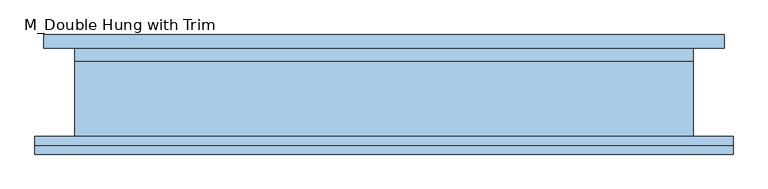
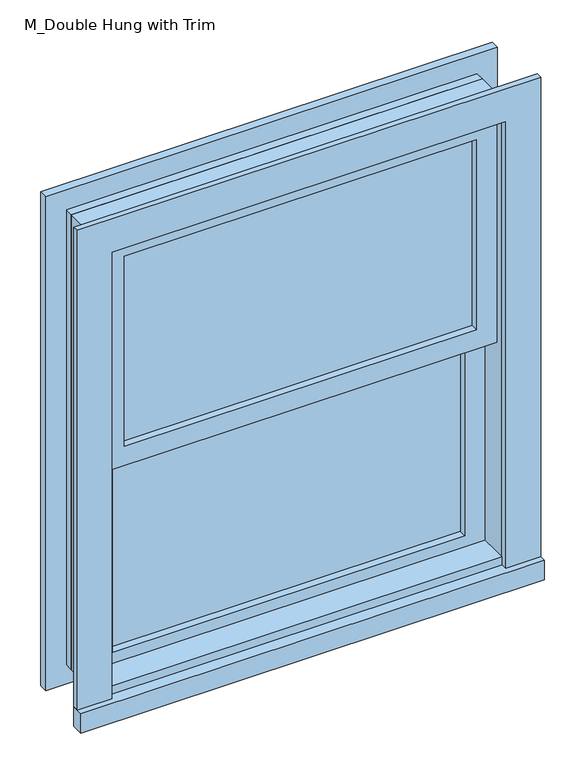
"""IFC4 building model written with IfcOpenShell, lengths in millimetres: window geometry, M_Double Hung with Trim."""

from ifc_helpers import new_model, si_unit, frame, origin, place, context, project, spatial, polyline, outline, extrude, source, transform, mapped, element, save


def m_double_hung_with_trim_e19062af(model_context):
    return source(origin(), model_context, "Body", "SweptSolid", [
        extrude(outline(polyline([(-381.0, 15.825), (-381.0, 28.525), (381.0, 28.525), (381.0, 15.825), (-381.0, 15.825)])), frame((0.0, 0.0, 628.65), z_axis=(0.0, 0.0, 1.0), x_axis=(1.0, 0.0, 0.0)), (0.0, 0.0, 1.0), 454.025),
        extrude(outline(polyline([(1127.125, -425.45), (584.2, -425.45), (584.2, 425.45), (1127.125, 425.45), (1127.125, -425.45)]), holes=[polyline([(1082.675, -381.0), (1082.675, 381.0), (628.65, 381.0), (628.65, -381.0), (1082.675, -381.0)])]), frame((0.0, -0.05, 0.0), z_axis=(0.0, 1.0, 0.0), x_axis=(0.0, 0.0, 1.0)), (0.0, 0.0, 1.0), 44.45),
        extrude(outline(polyline([(-501.65, -89.2), (-501.65, -63.5), (501.65, -63.5), (501.65, -89.2), (-501.65, -89.2)])), frame((0.0, 0.0, 539.75), z_axis=(0.0, 0.0, 1.0), x_axis=(1.0, 0.0, 0.0)), (0.0, 0.0, 1.0), 44.45),
        extrude(outline(polyline([(1682.75, -501.65), (539.75, -501.65), (539.75, 501.65), (1682.75, 501.65), (1682.75, -501.65)]), holes=[polyline([(1606.55, -425.45), (1606.55, 425.45), (584.2, 425.45), (584.2, -425.45), (1606.55, -425.45)])]), frame((0.0, -76.5, 0.0), z_axis=(0.0, 1.0, 0.0), x_axis=(0.0, 0.0, 1.0)), (0.0, 0.0, 1.0), 13.0),
        extrude(outline(polyline([(1670.05, 488.95), (1670.05, -488.95), (539.75, -488.95), (539.75, 488.95), (1670.05, 488.95)]), holes=[polyline([(1593.85, 412.75), (615.95, 412.75), (615.95, -412.75), (1593.85, -412.75), (1593.85, 412.75)])]), frame((0.0, 63.5, 0.0), z_axis=(0.0, 1.0, 0.0), x_axis=(0.0, 0.0, 1.0)), (0.0, 0.0, 1.0), 19.0),
        extrude(outline(polyline([(381.0, -15.925), (381.0, -28.625), (-381.0, -28.625), (-381.0, -15.925), (381.0, -15.925)])), frame((0.0, 0.0, 1127.125), z_axis=(0.0, 0.0, 1.0), x_axis=(1.0, 0.0, 0.0)), (0.0, 0.0, 1.0), 434.975),
        extrude(outline(polyline([(1606.55, -425.45), (1082.675, -425.45), (1082.675, 425.45), (1606.55, 425.45), (1606.55, -425.45)]), holes=[polyline([(1562.1, -381.0), (1562.1, 381.0), (1127.125, 381.0), (1127.125, -381.0), (1562.1, -381.0)])]), frame((0.0, -44.5, 0.0), z_axis=(0.0, 1.0, 0.0), x_axis=(0.0, 0.0, 1.0)), (0.0, 0.0, 1.0), 44.45),
        extrude(outline(polyline([(1625.6, -444.5), (584.2, -444.5), (584.2, 444.5), (1625.6, 444.5), (1625.6, -444.5)]), holes=[polyline([(1593.85, -412.75), (1593.85, 412.75), (615.95, 412.75), (615.95, -412.75), (1593.85, -412.75)])]), frame((0.0, 44.4, 0.0), z_axis=(0.0, 1.0, 0.0), x_axis=(0.0, 0.0, 1.0)), (0.0, 0.0, 1.0), 19.1),
        extrude(outline(polyline([(1625.6, 444.5), (1625.6, -444.5), (584.2, -444.5), (584.2, 444.5), (1625.6, 444.5)]), holes=[polyline([(1606.55, 425.45), (603.25, 425.45), (603.25, -425.45), (1606.55, -425.45), (1606.55, 425.45)])]), frame((0.0, -63.5, 0.0), z_axis=(0.0, 1.0, 0.0), x_axis=(0.0, 0.0, 1.0)), (0.0, 0.0, 1.0), 107.9),
    ])


if __name__ == "__main__":
    model = new_model("IFC4")
    model_context = context("Model", 3, world=origin())
    ifc_project = project(units=[si_unit("LENGTHUNIT", "METRE", prefix="MILLI")], contexts=[model_context])
    site = spatial("IfcSite", under=ifc_project)
    building = spatial("IfcBuilding", under=site)
    placement = place(None, origin())
    m_double_hung_with_trim_shape = m_double_hung_with_trim_e19062af(model_context)
    element("IfcWindow", 1, ObjectType="M_Double Hung with Trim : 2'  11\" x 3'  5\"", at=placement, inside=building, context=model_context, shape_type="MappedRepresentation", body=[
        mapped(m_double_hung_with_trim_shape, transform((0.0, 0.0, 0.0), x_axis=(1.0, 0.0, 0.0), y_axis=(0.0, 1.0, 0.0), z_axis=(0.0, 0.0, 1.0))),
    ])
    save(model, "model.ifc")

# Revit data of these elements
# Type "M_Double Hung with Trim : 2'  11\" x 3'  5\""
#   Type Mark = "72"
#   Construction Type Id = "GSP4R"
#   Analytic Construction = "1/8 in Pilkington single glazing"
#   Visual Light Transmittance = 0.9
#   Thermal Resistance (R) = 0.271106 (m²·K)/W
#   Solar Heat Gain Coefficient = 0.78
#   Heat Transfer Coefficient (U) = 3.6886 W/(m²·K)
#   Height = 3' - 5"
#   Default Sill Height = 1' - 11"
#   Trim Projection - Ext. = 0' - 0.51181"
#   Trim Projection - Int. = 0' - 0.74803"
#   Trim Width - Exterior = 0' - 3"
#   Trim Width - Interior = 0' - 3"
#   Width = 2' - 11"
#   Window Inset = 0' - 0.74803"
#   Glass Pane Material = EXISTING WINDOW
#   Sash = Trim
#   Trim Exterior Material = Trim
#   Trim Interior Material = Trim
#   Wall Closure = (empty or 0)
# Element 1 (IfcWindow, "M_Double Hung with Trim : 2'  11\" x 3'  5\"")
#   Materials on its faces: "Trim", "EXISTING WINDOW"
# Materials
#   "EXISTING WINDOW": class "Glass", colour RGB 218 227 224, transparency 0.85, Description = "Soda Lime Glass", Cost = 0
#   "Trim": class "Wood", colour RGB 250 251 245, transparency 0, Cost = 0
